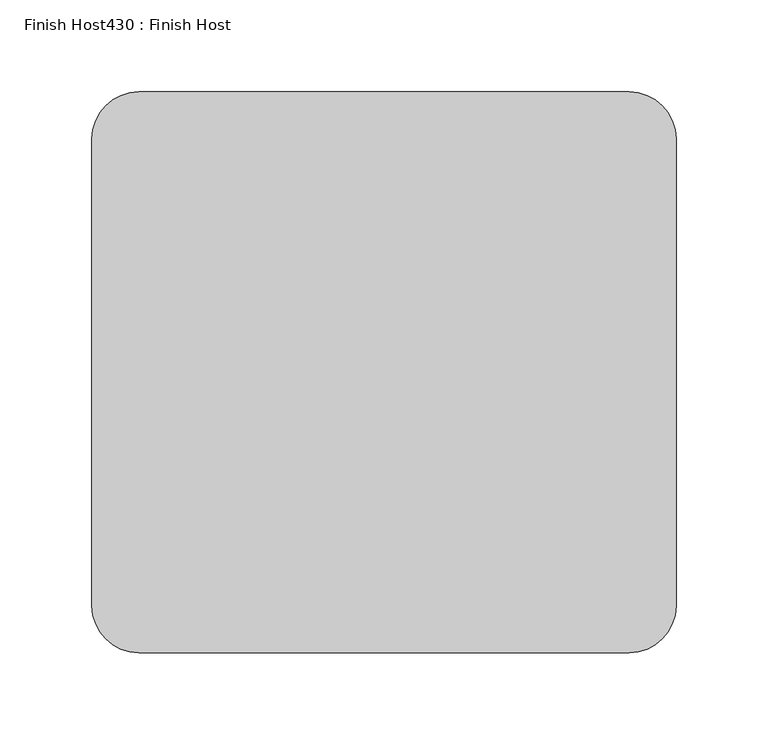
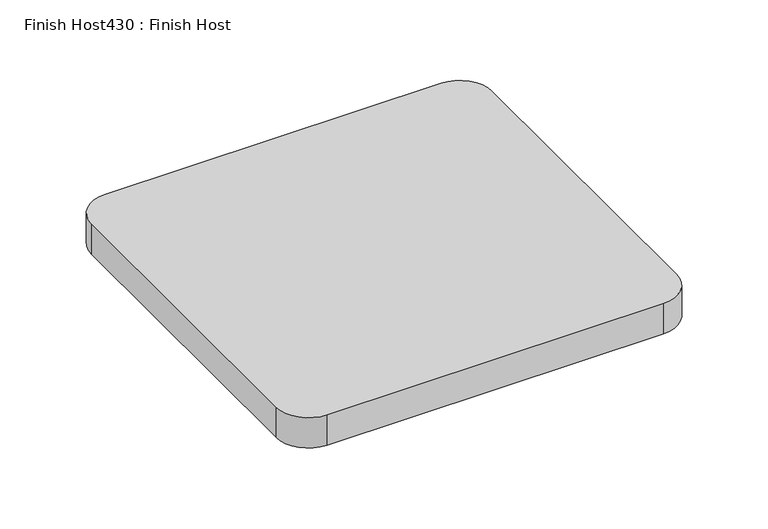
"""IFC4 building model written with IfcOpenShell, lengths in millimetres: proxy geometry, Finish Host430 : Finish Host."""

from ifc_helpers import new_model, si_unit, point, frame_2d, origin, origin_with_axes, place, context, project, spatial, polyline, circle_curve, trimmed, segment, composite_curve, outline, extrude, source, transform, mapped, element, save


def finish_host430_finish_host_c5fe1471(model_context):
    return source(origin(), model_context, "Body", "SweptSolid", [
        extrude(outline(composite_curve([segment(polyline([(-47.8842816, 4661.2760864), (-47.8842816, 4915.2760864)]), True, "CONTINUOUS"), segment(trimmed(circle_curve(frame_2d((-22.4842816, 4915.2760864)), 25.4), [point((-47.8842816, 4915.2760864))], [point((-22.4842816, 4940.6760864))], False, "CARTESIAN"), True, "CONTINUOUS"), segment(polyline([(-22.4842816, 4940.6760864), (244.2157184, 4940.6760864)]), True, "CONTINUOUS"), segment(trimmed(circle_curve(frame_2d((244.2157184, 4915.2760864)), 25.4), [point((244.2157184, 4940.6760864))], [point((269.6157184, 4915.2760864))], False, "CARTESIAN"), True, "CONTINUOUS"), segment(polyline([(269.6157184, 4915.2760864), (269.6157184, 4661.2760864)]), True, "CONTINUOUS"), segment(trimmed(circle_curve(frame_2d((244.2157184, 4661.2760864)), 25.4), [point((269.6157184, 4661.2760864))], [point((244.2157184, 4635.8760864))], False, "CARTESIAN"), True, "CONTINUOUS"), segment(polyline([(244.2157184, 4635.8760864), (-22.4842816, 4635.8760864)]), True, "CONTINUOUS"), segment(trimmed(circle_curve(frame_2d((-22.4842816, 4661.2760864)), 25.4), [point((-22.4842816, 4635.8760864))], [point((-47.8842816, 4661.2760864))], False, "CARTESIAN"), True, "CONTINUOUS")], self_intersect=False)), origin_with_axes(), (0.0, 0.0, 1.0), 25.4),
    ])


if __name__ == "__main__":
    model = new_model("IFC4")
    model_context = context("Model", 3, world=origin())
    ifc_project = project(units=[si_unit("LENGTHUNIT", "METRE", prefix="MILLI")], contexts=[model_context])
    site = spatial("IfcSite", under=ifc_project)
    building = spatial("IfcBuilding", under=site)
    placement = place(None, origin())
    finish_host430_finish_host_shape = finish_host430_finish_host_c5fe1471(model_context)
    element("IfcBuildingElementProxy", 1, Name="Finish Host430 : Finish Host", ObjectType="Finish Host430 : Finish Host", at=placement, inside=building, context=model_context, shape_type="MappedRepresentation", body=[
        mapped(finish_host430_finish_host_shape, transform((0.0, 0.0, 0.0), x_axis=(1.0, 0.0, 0.0), y_axis=(0.0, 1.0, 0.0), z_axis=(0.0, 0.0, 1.0))),
    ])
    save(model, "model.ifc")

# Revit data of these elements
# Type "Finish Host430 : Finish Host"
#   Countertop Material = Paint - Teknion - Accent - Crimson
# Element 1 (IfcBuildingElementProxy, "Finish Host430 : Finish Host")
#   Materials on its faces: "Paint - Teknion - Accent - Crimson"
# Materials
#   "Paint - Teknion - Accent - Crimson": class "Paint", colour RGB 131 56 52, transparency 0, Manufacturer = "Teknion", URL = "http://www.teknion.com/", Description = "Crimson", Cost = 0
